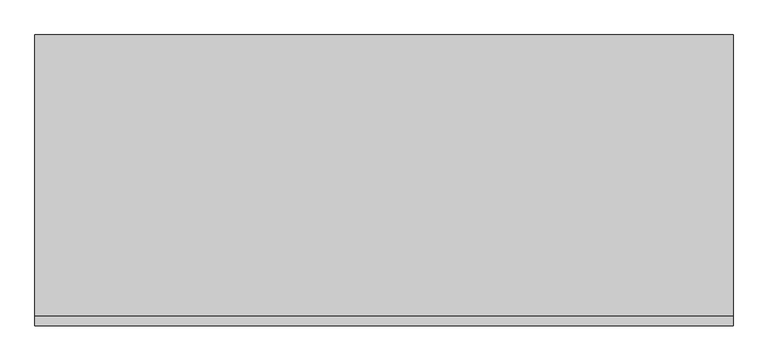
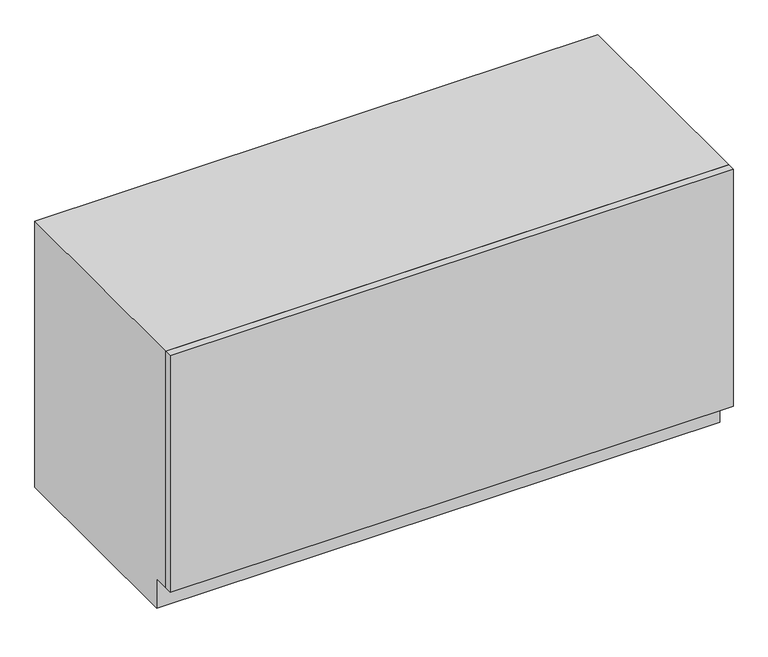
"""IFC4 building model written with IfcOpenShell, lengths in millimetres: furniture geometry, OD_CW_Base Cabinet : OD_CW_Base Cabinet."""

from ifc_helpers import new_model, si_unit, frame, origin, place, context, project, spatial, polyline, outline, extrude, source, transform, mapped, element, save


def furniture_fa5495af(model_context):
    return source(origin(), model_context, "Body", "SweptSolid", [
        extrude(outline(polyline([(18.7377049, -127.0), (1847.5377049, -127.0), (1847.5377049, -152.4), (18.7377049, -152.4), (18.7377049, -127.0)])), frame((0.0, 0.0, 101.6), z_axis=(0.0, 0.0, 1.0), x_axis=(1.0, 0.0, 0.0)), (0.0, 0.0, 1.0), 812.8),
        extrude(outline(polyline([(-127.0, 914.4), (609.6, 914.4), (609.6, 0.0), (-76.2, 0.0), (-76.2, 101.6), (-127.0, 101.6), (-127.0, 914.4)])), frame((18.7377049, 0.0, 0.0), z_axis=(1.0, 0.0, 0.0), x_axis=(0.0, 1.0, 0.0)), (0.0, 0.0, 1.0), 1828.8),
    ])


if __name__ == "__main__":
    model = new_model("IFC4")
    model_context = context("Model", 3, world=origin())
    ifc_project = project(units=[si_unit("LENGTHUNIT", "METRE", prefix="MILLI")], contexts=[model_context])
    site = spatial("IfcSite", under=ifc_project)
    building = spatial("IfcBuilding", under=site)
    placement = place(None, origin())
    furniture_shape = furniture_fa5495af(model_context)
    element("IfcFurniture", 1, ObjectType="OD_CW_Base Cabinet : OD_CW_Base Cabinet", at=placement, inside=building, context=model_context, shape_type="MappedRepresentation", body=[
        mapped(furniture_shape, transform((0.0, 0.0, 0.0), x_axis=(1.0, 0.0, 0.0), y_axis=(0.0, 1.0, 0.0), z_axis=(0.0, 0.0, 1.0))),
    ])
    save(model, "model.ifc")

# Revit data of these elements
# Type "OD_CW_Base Cabinet : OD_CW_Base Cabinet"
#   OD_CW_Width [instance default] = 2' - 10"
#   OD_CW_Length [instance default] = 8' - 0"
#   OD_CW_Height [instance default] = 2' - 3"
#   Depth = 2' - 0"
#   Height = 3' - 0"
#   Width = 4' - 0"
#   OD_CW_Material_Front Panel [instance default] = none
#   OD_CW_Material_Body [instance default] = none
# Element 1 (IfcFurniture, "OD_CW_Base Cabinet : OD_CW_Base Cabinet")
#   OD_CW_Width = 2' - 6"
#   OD_CW_Length = 6' - 0"
#   OD_CW_Height = 3' - 0"
#   OD_CW_Material_Body = PREP TABLE
#   Materials on its faces: "PREP TABLE", "CASEWORK"
# Materials
#   "PREP TABLE": class "Generic", colour RGB 187 187 187, transparency 0, Cost = 0
#   "CASEWORK": class "Generic", colour RGB 181 181 181, transparency 0, Cost = 0
